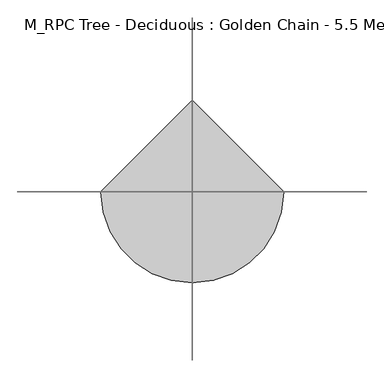
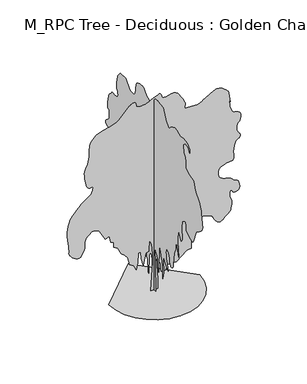
"""IFC4 building model written with IfcOpenShell, lengths in millimetres: geographic element geometry, M_RPC Tree - Deciduous : Golden Chain - 5.5 Meters."""

from ifc_helpers import new_model, si_unit, origin, place, context, project, spatial, triangles, source, transform, mapped, element, save


def m_rpc_tree_deciduous_golden_chain_5_5_meters_6778af60(model_context):
    return source(origin(), model_context, "Body", "Tessellation", [
        triangles([(-0.0021492, 84.2526153, 0.0017055), (-0.0021492, -79.7118042, 0.0017055), (-0.0021492, -55.1171299, 770.634066), (-0.0021492, -30.52271, 1205.1391577), (-0.0021492, -128.9011618, 1090.3648407), (-0.0021492, -161.6941456, 983.7870438), (-0.0021492, -161.6941456, 778.8331295), (-0.0021492, -202.6851937, 614.8669024), (-0.0021492, -227.2798771, 1410.0956154), (-0.0021492, -292.8648273, 1254.3285244), (-0.0021492, -391.2435245, 934.5977497), (-0.0021492, -407.6416878, 557.4810519), (-0.0021492, -448.6319547, 754.2384825), (-0.0021492, -424.0372713, 1123.1586239), (-0.0021492, -399.4426243, 1229.7338047), (-0.0021492, -563.4062716, 1024.7798904), (-0.0021492, -645.3893852, 910.00303), (-0.0021492, -571.6053351, 1164.1488544), (-0.0021492, -566.3701532, 1202.7023878), (-0.0021492, -561.3514189, 1240.6803749), (-0.0021492, -556.7629998, 1277.5125744), (-0.0021492, -552.8187638, 1312.6233673), (-0.0021492, -549.7351948, 1345.442585), (-0.0021492, -547.7261604, 1375.3895943), (-0.0021492, -547.0106518, 1401.8965519), (-0.0021492, -548.2048739, 1425.0576382), (-0.0021492, -551.550709, 1445.6369053), (-0.0021492, -556.6891308, 1464.0644142), (-0.0021492, -563.2636931, 1480.7706619), (-0.0021492, -570.9127539, 1496.1884708), (-0.0021492, -579.2773232, 1510.7457218), (-0.0021492, -588.000955, 1524.870005), (-0.0021492, -615.9185097, 1493.2475166), (-0.0021492, -642.6877333, 1461.6276443), (-0.0021492, -667.1627655, 1430.0051559), (-0.0021492, -688.1976734, 1398.3826675), (-0.0021492, -704.6416552, 1366.7627953), (-0.0021492, -715.3488504, 1335.1403069), (-0.0021492, -719.173399, 1303.5178185), (-0.0021492, -720.8463346, 1273.0922047), (-0.0021492, -725.5315138, 1244.8155876), (-0.0021492, -732.7248247, 1218.3340645), (-0.0021492, -741.9270973, 1193.2836313), (-0.0021492, -752.6342926, 1169.31024), (-0.0021492, -764.3472404, 1146.0549007), (-0.0021492, -776.5592857, 1123.1586239), (-0.0021492, -799.2416948, 1123.4208899), (-0.0021492, -820.9921841, 1125.2618385), (-0.0021492, -840.8787609, 1130.2576818), (-0.0021492, -857.9695055, 1139.9845591), (-0.0021492, -871.3298819, 1156.0210802), (-0.0021492, -880.0305862, 1179.9486168), (-0.0021492, -883.1370827, 1213.3382212), (-0.0021492, -884.8100183, 1255.5711811), (-0.0021492, -889.4951975, 1304.2589069), (-0.0021492, -896.6884357, 1358.3243568), (-0.0021492, -905.890781, 1416.6930325), (-0.0021492, -916.5979763, 1478.2854939), (-0.0021492, -928.3109241, 1542.0320389), (-0.0021492, -940.5255129, 1606.8530823), (-0.0021492, -1006.1104631, 1762.6177025), (-0.0021492, -1030.7051102, 2041.3581013), (-0.0021492, -1137.2829071, 1615.0495296), (-0.0021492, -1096.2900604, 2033.1590378), (-0.0021492, -1120.8847801, 2385.6835957), (-0.0021492, -1260.2563602, 2139.7368347), (-0.0021492, -1270.7241806, 2153.8611179), (-0.0021492, -1280.7616493, 2168.4183689), (-0.0021492, -1289.9410309, 2183.833707), (-0.0021492, -1297.8295029, 2200.5424255), (-0.0021492, -1303.9940975, 2218.9699345), (-0.0021492, -1308.0095501, 2239.5492016), (-0.0021492, -1309.4456543, 2262.7102879), (-0.0021492, -1307.6275967, 2290.0778034), (-0.0021492, -1302.9424175, 2322.033847), (-0.0021492, -1296.538448, 2357.1447853), (-0.0021492, -1289.5590775, 2393.9769848), (-0.0021492, -1283.1526371, 2431.0968121), (-0.0021492, -1278.467458, 2467.0683083), (-0.0021492, -1276.6518711, 2500.45784), (-0.0021492, -1277.8461296, 2532.7959824), (-0.0021492, -1281.1944717, 2566.4375336), (-0.0021492, -1286.3329662, 2601.1435547), (-0.0021492, -1292.9049488, 2636.6899315), (-0.0021492, -1300.5540459, 2672.8981865), (-0.0021492, -1308.9185062, 2709.5395546), (-0.0021492, -1317.642247, 2746.4096878), (-0.0021492, -1349.0965771, 2763.5973015), (-0.0021492, -1379.5477707, 2778.4931946), (-0.0021492, -1407.98993, 2788.7800667), (-0.0021492, -1433.4222439, 2792.1923584), (-0.0021492, -1454.8366344, 2786.4374771), (-0.0021492, -1471.2347614, 2769.1992851), (-0.0021492, -1481.6057854, 2738.2107697), (-0.0021492, -1484.4041611, 2701.900486), (-0.0021492, -1481.8935585, 2669.6135033), (-0.0021492, -1478.8100258, 2640.3309883), (-0.0021492, -1479.8871403, 2613.0602692), (-0.0021492, -1489.8532471, 2586.7825127), (-0.0021492, -1513.444685, 2560.5300453), (-0.0021492, -1555.3924152, 2533.2517685), (-0.0021492, -1606.8988644, 2505.0718025), (-0.0021492, -1655.253035, 2478.4681938), (-0.0021492, -1699.3015091, 2456.025087), (-0.0021492, -1737.903368, 2440.3219757), (-0.0021492, -1769.9076645, 2433.9411152), (-0.0021492, -1794.1662128, 2439.4615631), (-0.0021492, -1809.5357689, 2459.4676094), (-0.0021492, -1957.1037964, 2820.1761154), (-0.0021492, -2096.4727604, 2918.5648773), (-0.0021492, -2133.9033245, 2947.2108032), (-0.0021492, -2168.0337994, 2976.9770096), (-0.0021492, -2197.5760368, 3008.067263), (-0.0021492, -2221.2386913, 3040.5580124), (-0.0021492, -2237.731144, 3074.6530243), (-0.0021492, -2245.7620491, 3110.453746), (-0.0021492, -2244.0407879, 3148.1136566), (-0.0021492, -2235.2459759, 3194.9398682), (-0.0021492, -2223.869054, 3254.6760475), (-0.0021492, -2211.3438011, 3322.1530334), (-0.0021492, -2199.1063213, 3392.2013741), (-0.0021492, -2188.5901028, 3459.67836), (-0.0021492, -2181.2287788, 3519.4145393), (-0.0021492, -2178.4558376, 3566.2154617), (-0.0021492, -2170.3281361, 3608.6875786), (-0.0021492, -2147.5744377, 3658.060437), (-0.0021492, -2112.6315125, 3713.1367264), (-0.0021492, -2067.9338047, 3772.8217461), (-0.0021492, -2015.9257874, 3835.9446373), (-0.0021492, -1959.038998, 3901.3845383), (-0.0021492, -1899.7152935, 3967.9447197), (-0.0021492, -1842.3294067, 4197.4932083), (-0.0021492, -1629.1739582, 4246.6875893), (-0.0021492, -1457.0136818, 4328.652935), (-0.0021492, -1458.3505188, 4335.1970123), (-0.0021492, -1461.6963902, 4352.7409996), (-0.0021492, -1466.0480141, 4378.3565872), (-0.0021492, -1470.3970219, 4408.9631493), (-0.0021492, -1473.7428932, 4441.6065056), (-0.0021492, -1475.082201, 4473.2060303), (-0.0021492, -1473.409338, 4500.8334137), (-0.0021492, -1467.7438408, 4526.8565346), (-0.0021492, -1458.2079403, 4555.4515915), (-0.0021492, -1445.4433125, 4586.2107605), (-0.0021492, -1430.0993362, 4618.7015099), (-0.0021492, -1412.8176876, 4652.4654373), (-0.0021492, -1394.2474548, 4687.1205894), (-0.0021492, -1375.0306046, 4722.1829842), (-0.0021492, -1342.2368214, 4918.9352188), (-0.0021492, -1448.8146183, 5009.1250626), (-0.0021492, -1579.9871349, 4984.5277267), (-0.0021492, -1653.7685326, 4877.9400467), (-0.0021492, -1653.7685326, 4976.3288086), (-0.0021492, -1538.9942883, 5082.8914902), (-0.0021492, -1350.4358849, 5107.488826), (-0.0021492, -1202.8678574, 5074.692572), (-0.0021492, -1055.2998299, 5156.6829163), (-0.0021492, -948.7220329, 5164.8818344), (-0.0021492, -940.8819592, 5161.1390396), (-0.0021492, -920.1372952, 5151.1065125), (-0.0021492, -890.6409851, 5136.4911255), (-0.0021492, -856.5588358, 5118.9980072), (-0.0021492, -822.0437914, 5100.3334488), (-0.0021492, -791.2590425, 5082.280481), (-0.0021492, -768.3627657, 5066.4930725), (-0.0021492, -752.5400396, 5050.8591431), (-0.0021492, -739.1541561, 5033.7985565), (-0.0021492, -726.6289759, 5017.8844116), (-0.0021492, -713.3882143, 5005.6874817), (-0.0021492, -697.8532614, 4999.805864), (-0.0021492, -678.4453617, 5002.8359116), (-0.0021492, -653.5859053, 5017.2989822), (-0.0021492, -627.1527803, 5039.5790176), (-0.0021492, -603.7294281, 5064.0234558), (-0.0021492, -582.814135, 5090.2247635), (-0.0021492, -563.9078762, 5117.8777267), (-0.0021492, -546.5090472, 5146.6253906), (-0.0021492, -530.1108839, 5176.0602219), (-0.0021492, -514.2169049, 5205.8775879), (-0.0021492, -415.8382078, 5410.8290314), (-0.0021492, -169.8924643, 5451.8242035), (-0.0021492, -163.845268, 5451.6713058), (-0.0021492, -147.6161895, 5450.6783432), (-0.0021492, -124.0728773, 5447.9540909), (-0.0021492, -96.0842423, 5442.6323227), (-0.0021492, -66.5181736, 5433.8985535), (-0.0021492, -38.2425694, 5420.8359787), (-0.0021492, -14.1260625, 5402.6295319), (-0.0021492, 3.3458589, 5384.2457703), (-0.0021492, 15.2248406, 5370.0373352), (-0.0021492, 23.9488607, 5358.0950409), (-0.0021492, 31.9557643, 5346.6114395), (-0.0021492, 41.6836339, 5333.6761826), (-0.0021492, 55.5706269, 5317.4306625), (-0.0021492, 76.0543103, 5296.0418518), (-0.0021492, 97.13535, 5271.2916183), (-0.0021492, 113.1971331, 5247.5349289), (-0.0021492, 127.2514169, 5226.7827072), (-0.0021492, 142.3091915, 5211.0464584), (-0.0021492, 161.3827366, 5202.3638489), (-0.0021492, 187.483033, 5202.6946426), (-0.0021492, 223.6221062, 5214.076506), (-0.0021492, 264.351397, 5233.7851868), (-0.0021492, 302.4974698, 5257.3889786), (-0.0021492, 338.4919115, 5284.2012955), (-0.0021492, 372.7676173, 5313.5855484), (-0.0021492, 405.7523409, 5344.9307281), (-0.0021492, 437.8763975, 5377.549086), (-0.0021492, 469.5675954, 5410.8290314), (-0.0021492, 492.466452, 5419.4860611), (-0.0021492, 515.7217913, 5427.3286057), (-0.0021492, 539.6951463, 5433.618338), (-0.0021492, 564.7456158, 5437.5396103), (-0.0021492, 591.2271026, 5438.3035172), (-0.0021492, 619.503756, 5435.1205719), (-0.0021492, 649.9294424, 5427.2268677), (-0.0021492, 681.4067362, 5417.9076691), (-0.0021492, 712.0259428, 5409.8610672), (-0.0021492, 740.9213448, 5401.4075134), (-0.0021492, 767.2373257, 5390.7895569), (-0.0021492, 790.1107115, 5376.3009064), (-0.0021492, 808.6833424, 5356.2364334), (-0.0021492, 822.0921896, 5328.8381058), (-0.0021492, 831.6764156, 5297.4679276), (-0.0021492, 839.5393805, 5266.5047012), (-0.0021492, 845.9687845, 5235.9240097), (-0.0021492, 851.2523283, 5205.5973724), (-0.0021492, 855.672698, 5175.5253708), (-0.0021492, 859.522681, 5145.5556885), (-0.0021492, 863.0824202, 5115.6877441), (-0.0021492, 868.5086151, 5085.9976959), (-0.0021492, 874.8667299, 5057.4029297), (-0.0021492, 883.0886845, 5030.9469864), (-0.0021492, 894.1065439, 5007.6989868), (-0.0021492, 908.8546263, 4988.7803741), (-0.0021492, 928.2625259, 4975.2085281), (-0.0021492, 953.2646336, 4968.1298904), (-0.0021492, 983.5706326, 4964.7940475), (-0.0021492, 1017.0340696, 4962.6296448), (-0.0021492, 1051.7859455, 4962.7313828), (-0.0021492, 1085.9648186, 4966.2962814), (-0.0021492, 1117.7069944, 4974.4446213), (-0.0021492, 1145.1458719, 4988.347261), (-0.0021492, 1166.4176113, 5009.1250626), (-0.0021492, 1187.9516893, 5037.6180908), (-0.0021492, 1215.2250246, 5071.5857849), (-0.0021492, 1244.9327316, 5107.4120865), (-0.0021492, 1273.7822788, 5141.5326782), (-0.0021492, 1298.4736496, 5170.3309204), (-0.0021492, 1315.7070454, 5190.2430771), (-0.0021492, 1322.1822315, 5197.6786697), (-0.0021492, 1576.328056, 5181.2802521), (-0.0021492, 1674.7067894, 5058.2941544), (-0.0021492, 1679.9878624, 5049.3057495), (-0.0021492, 1685.3426228, 5039.1203247), (-0.0021492, 1690.840107, 5026.4652832), (-0.0021492, 1696.5540024, 5010.1691849), (-0.0021492, 1702.550584, 4988.9838501), (-0.0021492, 1708.9086262, 4961.7134216), (-0.0021492, 1715.69702, 4927.1347183), (-0.0021492, 1722.2461842, 4888.9655365), (-0.0021492, 1727.9344997, 4851.6622902), (-0.0021492, 1732.907452, 4815.0465019), (-0.0021492, 1737.304858, 4779.0417229), (-0.0021492, 1741.2720577, 4743.4444771), (-0.0021492, 1744.9539551, 4708.1530266), (-0.0021492, 1748.4908031, 4672.9886032), (-0.0021492, 1731.0893944, 4648.3403984), (-0.0021492, 1714.6937382, 4623.4122688), (-0.0021492, 1700.3046455, 4597.9237083), (-0.0021492, 1688.927869, 4571.5442139), (-0.0021492, 1681.5665451, 4544.0441483), (-0.0021492, 1679.2239555, 4515.0927177), (-0.0021492, 1682.9058529, 4484.4352867), (-0.0021492, 1691.9172215, 4457.546521), (-0.0021492, 1704.798848, 4438.9584114), (-0.0021492, 1721.4109154, 4426.9908279), (-0.0021492, 1741.6082291, 4419.8866104), (-0.0021492, 1765.2454491, 4415.940049), (-0.0021492, 1792.1827583, 4413.4445618), (-0.0021492, 1822.2748169, 4410.6435699), (-0.0021492, 1851.5776794, 4410.5162521), (-0.0021492, 1877.0099934, 4414.7177399), (-0.0021492, 1899.7152935, 4419.453788), (-0.0021492, 1920.8445271, 4421.0580505), (-0.0021492, 1941.543409, 4415.7871513), (-0.0021492, 1962.9576542, 4399.8982956), (-0.0021492, 1986.2385006, 4369.6483978), (-0.0021492, 2009.8529022, 4339.016256), (-0.0021492, 2031.6033188, 4320.2755394), (-0.0021492, 2051.6324741, 4307.2641243), (-0.0021492, 2070.0854176, 4293.8451759), (-0.0021492, 2087.1024021, 4273.8057014), (-0.0021492, 2102.8308025, 4241.0094475), (-0.0021492, 2117.4110172, 4189.2939995), (-0.0021492, 2130.4606567, 4132.1297562), (-0.0021492, 2141.5040234, 4085.4561516), (-0.0021492, 2150.5382103, 4046.6759605), (-0.0021492, 2157.565979, 4013.1922485), (-0.0021492, 2162.5848587, 3982.4330795), (-0.0021492, 2165.5945587, 3951.8009377), (-0.0021492, 2166.6003113, 3918.7500481), (-0.0021492, 2163.9699486, 3888.1437767), (-0.0021492, 2156.6086246, 3865.7361328), (-0.0021492, 2145.3030647, 3850.1274925), (-0.0021492, 2130.8426102, 3839.9676476), (-0.0021492, 2114.0167477, 3833.9075523), (-0.0021492, 2095.6120571, 3830.5464203), (-0.0021492, 2076.4181705, 3828.5602043), (-0.0021492, 2076.4181705, 3615.4098427), (-0.0021492, 2076.5861835, 3611.7687859), (-0.0021492, 2077.7574783, 3607.2362137), (-0.0021492, 2080.9351913, 3600.9979317), (-0.0021492, 2087.1278366, 3592.1877136), (-0.0021492, 2097.3334637, 3579.9143349), (-0.0021492, 2112.5576797, 3563.3636009), (-0.0021492, 2133.8065281, 3541.6437057), (-0.0021492, 2158.6890209, 3518.8288193), (-0.0021492, 2183.2835953, 3498.7640556), (-0.0021492, 2206.2996323, 3480.0997879), (-0.0021492, 2226.4484024, 3461.6134163), (-0.0021492, 2242.4391415, 3441.9561859), (-0.0021492, 2252.9807945, 3419.8796265), (-0.0021492, 2256.7799812, 3394.0602722), (-0.0021492, 2250.3276134, 3369.7687317), (-0.0021492, 2232.2566235, 3352.3773514), (-0.0021492, 2204.5070091, 3340.7152725), (-0.0021492, 2169.0142628, 3333.6366348), (-0.0021492, 2127.7106792, 3329.995578), (-0.0021492, 2082.5368378, 3328.6715309), (-0.0021492, 2035.4277946, 3328.4677643), (-0.0021492, 2021.5658501, 3329.995578), (-0.0021492, 2008.8496204, 3330.1737648), (-0.0021492, 1998.4275822, 3327.6274086), (-0.0021492, 1991.4508278, 3320.9815933), (-0.0021492, 1989.05984, 3308.886692), (-0.0021492, 1992.405566, 3289.9677887), (-0.0021492, 2002.6366276, 3262.9005455), (-0.0021492, 2020.3945553, 3234.9676575), (-0.0021492, 2044.3195484, 3213.2224731), (-0.0021492, 2072.5477673, 3195.7802238), (-0.0021492, 2103.212756, 3180.7570129), (-0.0021492, 2134.4508202, 3166.3195221), (-0.0021492, 2164.4003002, 3150.6088531), (-0.0021492, 2191.195031, 3131.7155296), (-0.0021492, 2214.6667088, 3115.4700096), (-0.0021492, 2235.4113728, 3106.0996513), (-0.0021492, 2252.7159851, 3099.4538361), (-0.0021492, 2265.8625664, 3091.381945), (-0.0021492, 2274.1329918, 3077.7083611), (-0.0021492, 2276.8091366, 3054.2824654), (-0.0021492, 2273.1754921, 3016.9539299), (-0.0021492, 2263.7593517, 2975.5765137), (-0.0021492, 2250.0398403, 2941.939904), (-0.0021492, 2232.735228, 2914.7709229), (-0.0021492, 2212.5634941, 2892.7455231), (-0.0021492, 2190.2375313, 2874.6158157), (-0.0021492, 2166.4806965, 2859.0580444), (-0.0021492, 2142.0055916, 2844.7731606), (-0.0021492, 2133.3761765, 2827.1783043), (-0.0021492, 2125.6812973, 2809.2779434), (-0.0021492, 2119.8477871, 2790.7918625), (-0.0021492, 2116.8125072, 2771.4654259), (-0.0021492, 2117.5051975, 2750.9675491), (-0.0021492, 2122.8599579, 2729.044178), (-0.0021492, 2133.8065281, 2705.4145157), (-0.0021492, 2153.6931049, 2682.9815826), (-0.0021492, 2182.4714355, 2663.4005104), (-0.0021492, 2215.980582, 2644.532476), (-0.0021492, 2250.062804, 2624.2386566), (-0.0021492, 2280.5623959, 2600.3543587), (-0.0021492, 2303.3160942, 2570.7407593), (-0.0021492, 2314.1683388, 2533.2517685), (-0.0021492, 2316.6306885, 2491.7827881), (-0.0021492, 2316.7960854, 2450.4562408), (-0.0021492, 2314.3822792, 2407.4085777), (-0.0021492, 2309.1012062, 2360.7782845), (-0.0021492, 2300.6627678, 2308.6964344), (-0.0021492, 2288.7842777, 2249.3015133), (-0.0021492, 2273.1754921, 2180.7272106), (-0.0021492, 2256.9479942, 2122.3126076), (-0.0021492, 2242.7269146, 2087.8459614), (-0.0021492, 2229.5091167, 2067.1470795), (-0.0021492, 2216.2913189, 2050.0334438), (-0.0021492, 2202.0702393, 2026.3248619), (-0.0021492, 2185.8401253, 1985.8335835), (-0.0021492, 2166.6003113, 1918.3847935), (-0.0021492, 2149.5808559, 1842.5203835), (-0.0021492, 2138.8736607, 1783.2936207), (-0.0021492, 2131.7517117, 1740.2713921), (-0.0021492, 2125.4903206, 1713.0234913), (-0.0021492, 2117.362619, 1701.1195667), (-0.0021492, 2104.6463894, 1704.1317375), (-0.0021492, 2084.617234, 1721.6273266), (-0.0021492, 2060.5012642, 1758.0775726), (-0.0021492, 2037.2458523, 1813.4570412), (-0.0021492, 2014.7060944, 1880.5977104), (-0.0021492, 1992.7391212, 1952.324437), (-0.0021492, 1971.2051159, 2021.4716698), (-0.0021492, 1949.9562675, 2080.8664455), (-0.0021492, 1928.8526138, 2123.3387077), (-0.0021492, 1903.2291779, 2154.4824463), (-0.0021492, 1869.4322582, 2184.7680977), (-0.0021492, 1828.8238358, 2214.3331535), (-0.0021492, 1782.7664726, 2243.3252792), (-0.0021492, 1732.6196789, 2271.8870533), (-0.0021492, 1679.7509583, 2300.1636703), (-0.0021492, 1625.51735, 2328.2952381), (-0.0021492, 1580.1042789, 2357.6693172), (-0.0021492, 1536.2697453, 2384.1049129), (-0.0021492, 1495.5901062, 2404.6612164), (-0.0021492, 1459.6414284, 2416.3971279), (-0.0021492, 1430.0025398, 2416.3715481), (-0.0021492, 1408.2521233, 2401.6489002), (-0.0021492, 1395.9662453, 2369.2854687), (-0.0021492, 1387.7442181, 2327.3633183), (-0.0021492, 1377.3731941, 2285.8713741), (-0.0021492, 1365.2069309, 2244.7359489), (-0.0021492, 1351.6071796, 2203.8882969), (-0.0021492, 1336.9303139, 2163.2544399), (-0.0021492, 1321.5379395, 2122.7657776), (-0.0021492, 1305.7865753, 2082.3484772), (-0.0021492, 1125.4248373, 1926.583857), (-0.0021492, 1107.9775738, 1907.1276318), (-0.0021492, 1091.2458916, 1886.8820652), (-0.0021492, 1075.9502409, 1865.0602867), (-0.0021492, 1062.8037323, 1840.8729549), (-0.0021492, 1052.5268887, 1813.5282578), (-0.0021492, 1045.8352186, 1782.2419407), (-0.0021492, 1043.4442308, 1746.2220463), (-0.0021492, 1042.7261787, 1711.1595062), (-0.0021492, 1040.7196878, 1682.5468632), (-0.0021492, 1037.6361551, 1659.3168858), (-0.0021492, 1033.6919191, 1640.3851925), (-0.0021492, 1029.1035364, 1624.6822266), (-0.0021492, 1024.0847294, 1611.1308735), (-0.0021492, 1018.8495838, 1598.6540188), (-0.0021492, 871.2814837, 1500.2752853), (-0.0021492, 854.8859001, 1328.1125381), (-0.0021492, 731.9125196, 1270.7241806), (-0.0021492, 699.1188091, 1057.5711302), (-0.0021492, 567.9463288, 1024.7798904), (-0.0021492, 579.9928319, 1019.3537682), (-0.0021492, 590.5345213, 1012.9956533), (-0.0021492, 598.0638946, 1004.7736261), (-0.0021492, 601.0736309, 993.7558393), (-0.0021492, 598.0638946, 979.0076843), (-0.0021492, 587.5222415, 959.5997847), (-0.0021492, 567.9463288, 934.5977497), (-0.0021492, 544.3090362, 908.8801334), (-0.0021492, 522.3905339, 887.4631994), (-0.0021492, 501.9081359, 869.6340551), (-0.0021492, 482.5715618, 854.6720324), (-0.0021492, 464.0956183, 841.8616224), (-0.0021492, 446.192605, 830.4822298), (-0.0021492, 428.5773285, 819.8234327), (-0.0021492, 416.3169213, 852.4974558), (-0.0021492, 404.2703819, 880.9396151), (-0.0021492, 392.6541942, 900.9203722), (-0.0021492, 381.6821895, 908.2104795), (-0.0021492, 371.5733952, 898.5777826), (-0.0021492, 362.5365921, 867.7931065), (-0.0021492, 354.7933147, 811.6243692), (-0.0021492, 347.289376, 757.5588467), (-0.0021492, 338.9222268, 728.4470335), (-0.0021492, 329.8396053, 713.1030573), (-0.0021492, 320.1840537, 700.3409729), (-0.0021492, 310.0981504, 678.9725098), (-0.0021492, 299.7245467, 637.8141209), (-0.0021492, 289.2083463, 565.677572), (-0.0021492, 280.1002358, 485.3215393), (-0.0021492, 273.5766333, 424.7553234), (-0.0021492, 269.2021002, 380.6814875), (-0.0021492, 266.5488464, 349.8000149), (-0.0021492, 265.1865749, 328.815976), (-0.0021492, 264.6849704, 314.426847), (-0.0021492, 264.613663, 303.3351912), (-0.0021492, 240.0187434, 811.6243692), (-0.0021492, 227.6618124, 844.6574547), (-0.0021492, 214.9461096, 875.6102165), (-0.0021492, 201.5133903, 902.4023312), (-0.0021492, 187.005355, 922.9585619), (-0.0021492, 171.062996, 935.1961143), (-0.0021492, 153.328032, 937.037063), (-0.0021492, 133.4419729, 926.401157), (-0.0021492, 115.707018, 904.291678), (-0.0021492, 103.9950694, 874.0085701), (-0.0021492, 97.3026454, 836.9141773), (-0.0021492, 94.6257194, 794.3680824), (-0.0021492, 94.9603011, 747.7377892), (-0.0021492, 97.3026454, 698.3803368), (-0.0021492, 100.6487348, 647.6606855), (-0.0021492, 84.2526153, 237.7499866), (88.4435659, 0.0002505, 0.0), (-86.3932913, 0.0002505, 0.0), (-44.7656723, 0.0002025, 807.5807934), (-36.4400473, 0.0001919, 1032.3704155), (-69.7422955, 0.0001759, 1307.1158546), (-128.0216733, 0.0001652, 1448.6490761), (-144.6726646, 0.0001865, 1140.6032713), (-227.9278935, 0.0001865, 1115.6266708), (-294.532658, 0.0002025, 799.2544121), (-352.8122947, 0.0001919, 999.0699772), (-361.138676, 0.0001812, 1182.2301636), (-427.7421324, 0.0001812, 1182.2301636), (-444.3923879, 0.0001972, 915.8137218), (-486.0217873, 0.0002079, 732.6509193), (-552.6252437, 0.0002025, 874.1842861), (-660.8581358, 0.0001972, 940.7903223), (-702.4849554, 0.0001812, 1157.2534904), (-785.7412107, 0.0001759, 1257.1625084), (-877.3238474, 0.0001759, 1332.0923824), (-977.2303219, 0.0001599, 1523.5789501), (-1085.4632504, 0.0001599, 1581.8586777), (-1085.4632504, 0.0001492, 1723.3945152), (-1160.3931244, 0.0001492, 1748.3711884), (-1202.019944, 0.0001386, 1939.857756), (-1318.5792538, 0.0001386, 1889.9044098), (-1468.4390018, 0.0001226, 2172.9736141), (-1502.3250149, 0.0001226, 2194.0442757), (-1536.1347244, 0.0001226, 2213.0727654), (-1569.8018555, 0.0001173, 2228.0246143), (-1603.2501045, 0.0001173, 2236.8602669), (-1636.4053482, 0.0001173, 2237.5401672), (-1669.1991314, 0.0001173, 2228.0246143), (-1701.5548599, 0.0001226, 2206.2766685), (-1733.4726791, 0.0001226, 2179.018594), (-1764.2269066, 0.0001226, 2153.3621658), (-1792.651189, 0.0001279, 2127.850787), (-1817.579464, 0.0001279, 2101.0306217), (-1837.8479942, 0.0001279, 2071.4426022), (-1852.2879559, 0.0001332, 2037.6304218), (-1859.7409893, 0.0001332, 1998.1373383), (-1862.0709343, 0.0001386, 1954.9318359), (-1863.0894768, 0.0001386, 1911.4359444), (-1864.5459286, 0.0001439, 1868.3754913), (-1868.1871307, 0.0001439, 1826.4812462), (-1875.759779, 0.0001439, 1786.4790367), (-1889.0133305, 0.0001492, 1749.0993416), (-1909.6943356, 0.0001492, 1715.0681339), (-1930.6655846, 0.0001546, 1683.7079842), (-1945.9586918, 0.0001546, 1654.8226833), (-1959.0644325, 0.0001546, 1629.87159), (-1973.4840466, 0.0001546, 1610.3057785), (-1992.7085999, 0.0001599, 1597.5870781), (-2020.2341, 0.0001599, 1593.1693245), (-2059.5539383, 0.0001599, 1598.5088242), (-2106.0849644, 0.0001546, 1614.4818317), (-2151.4523987, 0.0001546, 1639.6289886), (-2193.4662586, 0.0001546, 1671.9108845), (-2229.9496422, 0.0001492, 1709.2905796), (-2258.7125668, 0.0001492, 1749.7308437), (-2277.5730434, 0.0001439, 1791.1870342), (-2284.3435604, 0.0001439, 1831.6274437), (-2284.0049183, 0.0001439, 1867.2347179), (-2283.6662762, 0.0001386, 1899.34613), (-2284.3435604, 0.0001386, 1933.6447632), (-2287.0630165, 0.0001332, 1975.8062885), (-2292.8405708, 0.0001332, 2031.5116093), (-2302.6947659, 0.0001279, 2106.4440994), (-2317.6466148, 0.0001226, 2206.2766685), (-2328.3767738, 0.0001119, 2318.4664776), (-2327.0169731, 0.0001066, 2424.8304794), (-2316.773267, 0.0001013, 2522.6006744), (-2300.8512737, 9.59e-05, 2609.0116791), (-2282.4516701, 9.06e-05, 2681.301162), (-2264.780365, 9.06e-05, 2736.6829559), (-2251.0431221, 8.53e-05, 2772.4075195), (-2228.7604706, 8.53e-05, 2807.0370918), (-2187.9815643, 7.99e-05, 2856.639006), (-2135.6984184, 7.99e-05, 2914.8473717), (-2078.9007225, 7.46e-05, 2975.2454292), (-2024.5780209, 7.46e-05, 3031.4167099), (-1979.7200031, 6.93e-05, 3076.9444542), (-1951.3211552, 6.93e-05, 3105.4374825), (-1924.2819626, 6.4e-05, 3127.0812195), (-1882.823156, 6.4e-05, 3155.2940323), (-1832.9183533, 6.4e-05, 3188.4469505), (-1780.5385563, 5.86e-05, 3224.9607101), (-1731.6521507, 5.86e-05, 3263.2060501), (-1692.2328999, 5.33e-05, 3301.6042877), (-1668.2519508, 5.33e-05, 3338.5511604), (-1656.1646072, 5.33e-05, 3371.3218346), (-1648.0088551, 4.8e-05, 3398.84748), (-1643.1300831, 4.8e-05, 3421.9931602), (-1640.8716454, 4.8e-05, 3441.6759705), (-1640.5812561, 4.8e-05, 3458.7106865), (-1641.5997986, 4.8e-05, 3473.988533), (-1643.2752777, 4.26e-05, 3488.4260239), (-1673.4947994, 4.26e-05, 3483.4862091), (-1703.0597099, 4.26e-05, 3481.1180397), (-1731.3135086, 4.26e-05, 3483.8172935), (-1757.6014389, 4.26e-05, 3494.1806145), (-1781.2667095, 4.26e-05, 3514.7546494), (-1801.6574707, 4.26e-05, 3548.0601746), (-1818.1141697, 3.73e-05, 3596.6435463), (-1832.6281094, 3.2e-05, 3658.2386238), (-1846.5614159, 3.2e-05, 3726.3519081), (-1858.3075012, 2.66e-05, 3797.4190819), (-1866.2698059, 2.13e-05, 3867.7223488), (-1868.8440674, 1.6e-05, 3933.671521), (-1864.4261684, 1.6e-05, 3991.625251), (-1851.414608, 1.07e-05, 4037.8913223), (-1831.8514126, 1.07e-05, 4080.6180748), (-1810.1034668, 5.3e-06, 4129.8889046), (-1788.0628063, 5.3e-06, 4185.1436714), (-1767.626263, 0.0, 4245.7710754), (-1750.6831112, -5.3e-06, 4311.2106857), (-1739.1280025, -1.07e-05, 4380.8773636), (-1734.8579144, -1.07e-05, 4454.1853889), (-1735.4894165, -1.6e-05, 4523.877356), (-1735.8280586, -2.13e-05, 4584.5303398), (-1733.5466572, -2.13e-05, 4638.3334511), (-1726.3125057, -2.66e-05, 4687.5025429), (-1711.7987114, -3.2e-05, 4734.1761475), (-1687.6699516, -3.2e-05, 4780.5442474), (-1651.601659, -3.73e-05, 4828.8218239), (-1604.6581581, -3.73e-05, 4875.2407928), (-1551.3056007, -4.26e-05, 4914.6575729), (-1494.3144573, -4.26e-05, 4947.2247711), (-1436.4472046, -4.26e-05, 4973.1202835), (-1380.4746037, -4.26e-05, 4992.421431), (-1329.161602, -4.8e-05, 5005.3566879), (-1285.2761993, -4.8e-05, 5012.0022125), (-1238.819006, -4.8e-05, 5019.8197586), (-1181.7285227, -4.8e-05, 5034.7665207), (-1119.6854347, -4.8e-05, 5054.8059952), (-1058.3731888, -4.8e-05, 5077.9260956), (-1003.4673832, -5.33e-05, 5102.03974), (-960.651392, -5.33e-05, 5125.1598404), (-935.6009588, -5.33e-05, 5145.1993149), (-669.1845171, -6.93e-05, 5428.27099), (-646.0030106, -6.93e-05, 5444.1601364), (-622.8954094, -7.46e-05, 5458.928421), (-599.9328938, -7.46e-05, 5471.5328842), (-577.1893693, -7.46e-05, 5480.8520828), (-554.7386684, -7.46e-05, 5485.7918976), (-532.6495734, -7.46e-05, 5485.2826263), (-510.9983877, -7.46e-05, 5478.2295685), (-495.8275477, -7.46e-05, 5462.4933197), (-489.5407585, -6.93e-05, 5439.0418442), (-486.7500132, -6.93e-05, 5411.3888809), (-482.064834, -6.93e-05, 5382.9725922), (-470.0972506, -6.93e-05, 5357.3567139), (-445.4618357, -6.4e-05, 5337.9794083), (-402.7655319, -6.4e-05, 5328.3544144), (-352.1553217, -6.4e-05, 5326.9794983), (-306.7905035, -6.4e-05, 5329.5258545), (-265.7951497, -6.4e-05, 5335.3568939), (-228.2925333, -6.4e-05, 5343.8104477), (-193.4123404, -6.4e-05, 5354.2249283), (-160.2801876, -6.93e-05, 5365.9375854), (-128.0216733, -6.93e-05, 5378.3124115), (-76.4902348, -6.93e-05, 5408.3588333), (-26.1968067, -6.93e-05, 5436.7501236), (21.6206779, -7.46e-05, 5461.7805725), (65.7244948, -7.46e-05, 5481.7688873), (104.8766017, -7.46e-05, 5495.0605179), (137.8389157, -7.46e-05, 5500.0003326), (163.3739486, -7.46e-05, 5494.8820404), (179.7578323, -7.46e-05, 5482.2525787), (188.4231282, -7.46e-05, 5466.2872742), (192.8648993, -7.46e-05, 5447.6994553), (196.5786624, -6.93e-05, 5427.2012878), (203.0594986, -6.93e-05, 5405.5578415), (215.8026888, -6.93e-05, 5383.4562836), (238.3035501, -6.93e-05, 5361.6599396), (275.7078804, -6.4e-05, 5352.0093658), (327.5301169, -6.93e-05, 5359.8263306), (388.8194718, -6.93e-05, 5376.0974304), (454.6234131, -6.93e-05, 5391.7569397), (519.9893723, -6.93e-05, 5397.8426147), (579.9673974, -6.93e-05, 5385.2643127), (629.6048836, -6.4e-05, 5345.0068863), (669.510442, -6.4e-05, 5289.625383), (704.1731518, -5.86e-05, 5237.2989258), (734.4638901, -5.86e-05, 5187.5188248), (761.2611643, -5.33e-05, 5139.7758087), (785.4382496, -5.33e-05, 5093.5606064), (807.8660231, -4.8e-05, 5048.3633652), (829.420376, -4.8e-05, 5003.6759766), (821.0939947, -3.73e-05, 4853.8011131), (1104.163199, -3.73e-05, 4837.1483505), (1130.912075, -3.73e-05, 4839.0834068), (1157.5870457, -3.73e-05, 4841.7826607), (1184.116967, -3.73e-05, 4846.1111755), (1210.4303318, -3.73e-05, 4852.8334396), (1236.4509819, -3.73e-05, 4862.7639381), (1262.10741, -3.73e-05, 4876.6921577), (1287.3259289, -3.73e-05, 4895.433165), (1317.642247, -4.26e-05, 4918.5532654), (1357.5732399, -4.26e-05, 4944.7039948), (1405.5097034, -4.26e-05, 4973.4260788), (1459.8579849, -4.8e-05, 5004.1852478), (1519.010915, -4.8e-05, 5036.4722305), (1581.3671379, -4.8e-05, 5069.7527573), (1645.3250072, -5.33e-05, 5103.5675537), (1684.4540142, -5.33e-05, 5099.8497574), (1722.8521065, -5.33e-05, 5095.2663162), (1759.7963631, -5.33e-05, 5088.9515854), (1794.5558693, -4.8e-05, 5079.9887604), (1826.3998558, -4.8e-05, 5067.5371948), (1854.6051109, -4.8e-05, 5050.7062454), (1878.4410107, -4.8e-05, 5028.6552658), (1900.2143909, -4.8e-05, 5007.1897156), (1922.1329659, -4.26e-05, 4990.5372437), (1943.3232422, -4.26e-05, 4975.3358459), (1962.9118721, -4.26e-05, 4958.2502609), (1980.023037, -4.26e-05, 4935.9190659), (1993.7857143, -3.73e-05, 4905.0069992), (2003.3267017, -3.73e-05, 4862.1273491), (2036.62714, -2.13e-05, 4620.6877258), (2031.3358932, -2.66e-05, 4643.2223969), (2026.4088684, -2.66e-05, 4661.7340576), (2022.2099968, -2.66e-05, 4672.2502762), (2019.1035004, -2.66e-05, 4670.7477516), (2017.450985, -2.66e-05, 4653.2293442), (2017.6216141, -2.13e-05, 4615.6714622), (2019.9769936, -2.13e-05, 4554.0766754), (2029.0544918, -1.6e-05, 4483.8242775), (2046.7257969, -1.07e-05, 4423.1715843), (2069.3470905, -5.3e-06, 4372.5511276), (2093.2796413, -5.3e-06, 4332.4213097), (2114.8825378, -5.3e-06, 4303.2408234), (2130.5141418, -5.3e-06, 4285.3913315), (2136.5336872, 0.0, 4279.3565254), (2147.5539448, 0.0, 4280.1460121), (2175.7593452, 0.0, 4279.6367409), (2213.8671936, 0.0, 4273.4493279), (2254.5977016, 0.0, 4257.2038078), (2290.6659943, 0.0, 4226.5463768), (2314.794754, 5.3e-06, 4177.0973602), (2319.6963444, 1.07e-05, 4104.5023727), (2308.0216209, 1.07e-05, 4035.0650414), (2289.5024025, 1.6e-05, 3991.3959045), (2267.4871765, 1.6e-05, 3963.6159142), (2245.3241398, 1.6e-05, 3941.7939903), (2226.3694828, 2.13e-05, 3916.0255051), (2213.96399, 2.13e-05, 3876.4308289), (2211.466032, 2.66e-05, 3813.104171), (2219.5963497, 2.66e-05, 3747.2826073), (2234.7188278, 3.2e-05, 3702.4167412), (2253.6250866, 3.2e-05, 3671.9886566), (2273.1169201, 3.73e-05, 3649.4284058), (2289.9862392, 3.73e-05, 3628.141333), (2301.0320766, 3.73e-05, 3601.6598099), (2303.0461979, 4.26e-05, 3563.3380211), (2294.2843781, 4.26e-05, 3529.0395332), (2276.7837021, 4.26e-05, 3512.233873), (2253.0190189, 4.26e-05, 3502.8382256), (2225.4707005, 4.26e-05, 3490.8194824), (2196.6083633, 4.8e-05, 3466.1204086), (2168.9148502, 4.8e-05, 3418.7340569), (2144.8600685, 5.33e-05, 3338.5511604), (2129.882785, 5.86e-05, 3243.8796135), (2124.958231, 6.4e-05, 3160.284716), (2125.8545425, 6.93e-05, 3088.6321129), (2128.3549713, 7.46e-05, 3029.812738), (2128.2327404, 7.46e-05, 2984.6666565), (2121.2660145, 7.46e-05, 2954.0856743), (2103.2331036, 7.99e-05, 2938.9351456), (2080.3674934, 7.99e-05, 2933.5625084), (2059.979203, 7.99e-05, 2930.6853584), (2039.4433926, 7.99e-05, 2928.6482735), (2016.1421986, 7.99e-05, 2925.9237305), (1987.4504906, 7.99e-05, 2920.8565979), (1950.7506958, 7.99e-05, 2911.8426132), (1903.4176838, 7.99e-05, 2897.3033844), (1853.5127357, 7.99e-05, 2880.1413506), (1811.035532, 7.99e-05, 2862.9793167), (1776.2784966, 8.53e-05, 2843.7801979), (1749.5296932, 8.53e-05, 2820.5069092), (1731.0818367, 8.53e-05, 2791.0973671), (1721.2276417, 9.06e-05, 2753.5647743), (1720.2574974, 9.06e-05, 2705.8217583), (1723.631274, 9.59e-05, 2658.5115646), (1727.8785439, 9.59e-05, 2621.9722252), (1734.8910519, 9.59e-05, 2593.7338326), (1746.5683914, 0.0001013, 2571.3520592), (1764.7947498, 0.0001013, 2552.2802582), (1791.4723366, 0.0001013, 2534.1046234), (1828.4878098, 0.0001013, 2514.3224007), (1873.0047146, 0.0001013, 2496.0453186), (1919.5611752, 0.0001066, 2482.2824959), (1966.1151649, 0.0001066, 2470.414325), (2010.6320698, 0.0001066, 2457.815094), (2051.0697178, 0.0001066, 2441.8678116), (2085.3913147, 0.0001066, 2419.9517075), (2111.5570141, 0.0001119, 2389.4394711), (2135.660194, 0.0001119, 2361.79174), (2163.6949654, 0.0001119, 2345.6507195), (2193.4790485, 0.0001119, 2334.1695889), (2222.8250771, 0.0001119, 2320.5060333), (2249.5484459, 0.0001173, 2297.8084362), (2271.4670208, 0.0001173, 2259.2397148), (2286.3959061, 0.0001226, 2197.9502872), (2290.3019176, 0.0001279, 2132.9738754), (2281.9781525, 0.0001279, 2085.9081436), (2263.4563179, 0.0001279, 2053.7712971), (2236.7813473, 0.0001332, 2033.5767448), (2203.9875641, 0.0001332, 2022.3373146), (2167.1171402, 0.0001332, 2017.0716476), (2128.2097767, 0.0001332, 2014.7876301), (2106.9227039, 0.0001332, 2046.2216125), (2086.3639297, 0.0001279, 2073.5764835), (2067.2591366, 0.0001279, 2092.7780731), (2050.3415646, 0.0001279, 2099.7421829), (2036.3368961, 0.0001279, 2090.3972591), (2025.9709591, 0.0001279, 2060.6641903), (2019.9769936, 0.0001332, 2006.4637196), (2022.3322277, 0.0001386, 1947.8937481), (2033.7142365, 0.0001386, 1903.8861145), (2049.9035099, 0.0001439, 1868.6174824), (2066.6760326, 0.0001439, 1836.2616085), (2079.809824, 0.0001439, 1800.992831), (2085.075491, 0.0001492, 1756.9878136), (2078.2539597, 0.0001492, 1698.4178421), (2066.069965, 0.0001546, 1638.7046265), (2056.21577, 0.0001599, 1592.8306824), (2045.9236656, 0.0001599, 1557.2944794), (2032.4282684, 0.0001599, 1528.6053875), (2012.9618694, 0.0001652, 1503.2646378), (1984.7566143, 0.0001652, 1477.7762226), (1945.0471195, 0.0001652, 1448.6490761), (1902.3507431, 0.0001705, 1414.6917011), (1865.4803192, 0.0001705, 1379.8609783), (1832.1060482, 0.0001705, 1348.3784523), (1799.895369, 0.0001759, 1324.4688652), (1766.5210979, 0.0001759, 1312.3585579), (1729.6508194, 0.0001759, 1316.2645695), (1686.954443, 0.0001705, 1340.416293), (1647.1227173, 0.0001705, 1378.2109337), (1618.0669327, 0.0001705, 1418.4780979), (1596.2935524, 0.0001652, 1458.6025383), (1578.3090397, 0.0001652, 1495.9567989), (1560.6149162, 0.0001599, 1527.9254871), (1539.7148838, 0.0001599, 1551.8810017), (1512.115551, 0.0001599, 1565.2083858), (1471.7517357, 0.0001599, 1577.5375751), (1418.5696621, 0.0001599, 1596.5685356), (1358.1053295, 0.0001546, 1616.7632332), (1295.8943012, 0.0001546, 1632.58843), (1237.4695244, 0.0001546, 1638.511179), (1188.3667076, 0.0001546, 1628.9956261), (1154.1164726, 0.0001599, 1598.5088242), (1127.3931038, 0.0001599, 1577.4407787), (1098.3373192, 0.0001599, 1588.9958874), (1068.7009741, 0.0001546, 1616.8600296), (1040.2282934, 0.0001546, 1644.7266426), (1014.6711325, 0.0001546, 1656.2792805), (993.7711, 0.0001546, 1635.211235), (979.2801241, 0.0001599, 1565.2083858), (971.8780323, 0.0001652, 1477.5598114), (970.009033, 0.0001705, 1410.4444313), (972.0715525, 0.0001705, 1357.8940052), (976.4639442, 0.0001759, 1313.9347698), (981.5871054, 0.0001759, 1272.5981941), (985.8343025, 0.0001812, 1227.9132763), (987.6065054, 0.0001812, 1173.9063257), (995.9303432, 0.0002025, 832.5574665), (871.0472683, 0.0002025, 807.5807934), (729.5139015, 0.0002132, 691.0215563), (587.9780276, 0.0002185, 591.1150818), (396.4889165, 0.0002185, 599.4414631), (329.8854238, 0.0002185, 557.8146071), (304.9088233, 0.0002238, 457.9055892), (278.3305583, 0.0002238, 452.8104424), (252.8434148, 0.0002238, 449.2405294), (229.5414941, 0.0002238, 448.7312582), (209.5163901, 0.0002238, 452.8104424), (193.8604962, 0.0002238, 463.0032432), (183.6658786, 0.0002238, 480.845141), (180.0249308, 0.0002238, 507.8588264), (179.9037354, 0.0002185, 542.6437672), (179.0540417, 0.0002185, 581.2125249), (176.7483685, 0.0002132, 621.2377344), (172.257963, 0.0002132, 660.3896324), (164.854872, 0.0002132, 696.3382376), (153.8105607, 0.0002079, 726.7512068), (138.3973209, 0.0002079, 749.3012112), (121.7702562, 0.0002079, 768.113217), (107.3279238, 0.0002079, 788.6719912), (94.7059289, 0.0002025, 810.6872898), (83.5404222, 0.0002025, 833.8687963), (73.4672725, 0.0002025, 857.9236507), (64.1223624, 0.0002025, 882.5590656), (55.1413199, 0.0001972, 907.4872679), (63.4669473, 0.0002132, 691.0215563), (88.4435659, 0.0002345, 266.4189852), (-1216.0703945, 0.0, 0.0051165), (-1183.9209034, -278.6437659, 0.0051165), (-1092.3611578, -534.5312536, 0.0051165), (-948.7220329, -760.3342587, 0.0051165), (-760.3342587, -948.7220329, 0.0051165), (-534.5312536, -1092.3611578, 0.0051165), (-278.6437659, -1183.9209034, 0.0051165), (5.32e-05, -1216.0703945, 0.0051165), (278.6437659, -1183.9209034, 0.0051165), (534.5312536, -1092.3611578, 0.0051165), (760.3342587, -948.7220329, 0.0051165), (948.7220329, -760.3342587, 0.0051165), (1092.3611578, -534.5312536, 0.0051165), (1183.9209034, -278.6437659, 0.0051165), (1216.0703945, 0.0001066, 0.0051165), (-0.0001595, 1216.0703945, 0.0051165)], [[476, 477, 478], [475, 476, 478], [474, 475, 478], [473, 474, 478], [62, 63, 64], [472, 473, 478], [471, 472, 478], [470, 471, 478], [11, 12, 13], [11, 13, 14], [7, 8, 9], [6, 7, 9], [16, 17, 18], [469, 470, 478], [5, 6, 9], [10, 11, 14], [10, 14, 15], [468, 469, 478], [151, 152, 153], [151, 153, 154], [15, 16, 18], [467, 468, 478], [150, 151, 154], [150, 154, 155], [4, 5, 9], [15, 18, 19], [65, 66, 67], [65, 67, 68], [65, 68, 69], [65, 69, 70], [65, 70, 71], [65, 71, 72], [65, 72, 73], [65, 73, 74], [65, 74, 75], [65, 75, 76], [65, 76, 77], [466, 467, 478], [465, 466, 478], [464, 465, 478], [463, 464, 478], [15, 19, 20], [455, 456, 457], [65, 77, 78], [149, 150, 155], [149, 155, 156], [15, 20, 21], [62, 64, 65], [1, 2, 3], [493, 1, 3], [492, 493, 3], [491, 492, 3], [490, 491, 3], [489, 490, 3], [489, 3, 4], [488, 489, 4], [487, 488, 4], [486, 487, 4], [485, 486, 4], [484, 485, 4], [462, 463, 478], [462, 478, 479], [65, 78, 79], [15, 21, 22], [462, 479, 480], [461, 462, 480], [461, 480, 481], [391, 392, 393], [454, 455, 457], [440, 441, 442], [15, 22, 23], [65, 79, 80], [391, 393, 394], [390, 391, 394], [390, 394, 395], [389, 390, 395], [389, 395, 396], [388, 389, 396], [388, 396, 397], [387, 388, 397], [387, 397, 398], [386, 387, 398], [386, 398, 399], [385, 386, 399], [385, 399, 400], [384, 385, 400], [131, 132, 133], [45, 46, 47], [438, 439, 440], [383, 384, 400], [383, 400, 401], [382, 383, 401], [381, 382, 401], [380, 381, 401], [379, 380, 401], [379, 401, 402], [378, 379, 402], [378, 402, 403], [377, 378, 403], [376, 377, 403], [376, 403, 404], [375, 376, 404], [374, 375, 404], [373, 374, 404], [372, 373, 404], [371, 372, 404], [370, 371, 404], [369, 370, 404], [368, 369, 404], [367, 368, 404], [367, 404, 405], [366, 367, 405], [366, 405, 406], [366, 406, 407], [365, 366, 407], [365, 407, 408], [365, 408, 409], [364, 365, 409], [364, 409, 410], [363, 364, 410], [363, 410, 411], [15, 23, 24], [10, 15, 24], [9, 10, 24], [9, 24, 25], [9, 25, 26], [9, 26, 27], [9, 27, 28], [9, 28, 29], [179, 180, 181], [454, 457, 458], [453, 454, 458], [452, 453, 458], [461, 481, 482], [452, 458, 459], [451, 452, 459], [250, 251, 252], [9, 29, 30], [65, 80, 81], [460, 461, 482], [249, 250, 252], [249, 252, 253], [248, 249, 253], [247, 248, 253], [246, 247, 253], [246, 253, 254], [246, 254, 255], [246, 255, 256], [246, 256, 257], [246, 257, 258], [246, 258, 259], [246, 259, 260], [245, 246, 260], [245, 260, 261], [244, 245, 261], [244, 261, 262], [244, 262, 263], [244, 263, 264], [243, 244, 264], [243, 264, 265], [243, 265, 266], [243, 266, 267], [243, 267, 268], [243, 268, 269], [243, 269, 270], [243, 270, 271], [243, 271, 272], [242, 243, 272], [242, 272, 273], [241, 242, 273], [362, 363, 411], [450, 451, 459], [362, 411, 412], [483, 484, 4], [9, 30, 31], [241, 273, 274], [240, 241, 274], [449, 450, 459], [449, 459, 460], [448, 449, 460], [447, 448, 460], [446, 447, 460], [445, 446, 460], [444, 445, 460], [443, 444, 460], [442, 443, 460], [361, 362, 412], [9, 31, 32], [65, 81, 82], [106, 107, 108], [105, 106, 108], [105, 108, 109], [104, 105, 109], [103, 104, 109], [102, 103, 109], [101, 102, 109], [100, 101, 109], [99, 100, 109], [98, 99, 109], [97, 98, 109], [96, 97, 109], [95, 96, 109], [94, 95, 109], [93, 94, 109], [92, 93, 109], [45, 47, 48], [44, 45, 48], [44, 48, 49], [44, 49, 50], [44, 50, 51], [44, 51, 52], [44, 52, 53], [43, 44, 53], [43, 53, 54], [42, 43, 54], [41, 42, 54], [40, 41, 54], [40, 54, 55], [39, 40, 55], [38, 39, 55], [38, 55, 56], [37, 38, 56], [37, 56, 57], [36, 37, 57], [36, 57, 58], [35, 36, 58], [35, 58, 59], [34, 35, 59], [33, 34, 59], [33, 59, 60], [32, 33, 60], [32, 60, 61], [32, 61, 62], [239, 240, 274], [179, 181, 182], [179, 182, 183], [179, 183, 184], [179, 184, 185], [179, 185, 186], [179, 186, 187], [179, 187, 188], [179, 188, 189], [179, 189, 190], [179, 190, 191], [179, 191, 192], [179, 192, 193], [179, 193, 194], [179, 194, 195], [179, 195, 196], [179, 196, 197], [179, 197, 198], [178, 179, 198], [177, 178, 198], [177, 198, 199], [176, 177, 199], [175, 176, 199], [174, 175, 199], [442, 460, 482], [442, 482, 483], [442, 483, 4], [440, 442, 4], [438, 440, 4], [438, 4, 9], [360, 361, 412], [239, 274, 275], [174, 199, 200], [173, 174, 200], [436, 437, 438], [435, 436, 438], [434, 435, 438], [433, 434, 438], [433, 438, 9], [432, 433, 9], [431, 432, 9], [430, 431, 9], [429, 430, 9], [428, 429, 9], [427, 428, 9], [426, 427, 9], [426, 9, 32], [426, 32, 62], [426, 62, 65], [425, 426, 65], [424, 425, 65], [423, 424, 65], [422, 423, 65], [421, 422, 65], [420, 421, 65], [419, 420, 65], [418, 419, 65], [417, 418, 65], [416, 417, 65], [415, 416, 65], [414, 415, 65], [414, 65, 82], [414, 82, 83], [414, 83, 84], [414, 84, 85], [414, 85, 86], [414, 86, 87], [413, 414, 87], [238, 239, 275], [359, 360, 412], [148, 149, 156], [148, 156, 157], [148, 157, 158], [148, 158, 159], [148, 159, 160], [148, 160, 161], [148, 161, 162], [148, 162, 163], [148, 163, 164], [148, 164, 165], [148, 165, 166], [148, 166, 167], [148, 167, 168], [148, 168, 169], [148, 169, 170], [147, 148, 170], [146, 147, 170], [145, 146, 170], [144, 145, 170], [143, 144, 170], [142, 143, 170], [141, 142, 170], [140, 141, 170], [139, 140, 170], [138, 139, 170], [137, 138, 170], [136, 137, 170], [135, 136, 170], [134, 135, 170], [134, 170, 171], [359, 412, 413], [359, 413, 87], [92, 109, 110], [324, 325, 326], [323, 324, 326], [323, 326, 327], [322, 323, 327], [321, 322, 327], [321, 327, 328], [320, 321, 328], [320, 328, 329], [319, 320, 329], [319, 329, 330], [318, 319, 330], [317, 318, 330], [317, 330, 331], [317, 331, 332], [316, 317, 332], [316, 332, 333], [315, 316, 333], [314, 315, 333], [314, 333, 334], [313, 314, 334], [312, 313, 334], [312, 334, 335], [311, 312, 335], [359, 87, 88], [237, 238, 275], [358, 359, 88], [357, 358, 88], [356, 357, 88], [355, 356, 88], [354, 355, 88], [353, 354, 88], [352, 353, 88], [351, 352, 88], [350, 351, 88], [349, 350, 88], [348, 349, 88], [347, 348, 88], [346, 347, 88], [345, 346, 88], [344, 345, 88], [343, 344, 88], [342, 343, 88], [341, 342, 88], [340, 341, 88], [339, 340, 88], [338, 339, 88], [337, 338, 88], [336, 337, 88], [335, 336, 88], [311, 335, 88], [310, 311, 88], [309, 310, 88], [309, 88, 89], [309, 89, 90], [172, 173, 200], [91, 92, 110], [91, 110, 111], [91, 111, 112], [91, 112, 113], [91, 113, 114], [91, 114, 115], [91, 115, 116], [91, 116, 117], [91, 117, 118], [91, 118, 119], [91, 119, 120], [91, 120, 121], [91, 121, 122], [91, 122, 123], [91, 123, 124], [91, 124, 125], [91, 125, 126], [91, 126, 127], [91, 127, 128], [91, 128, 129], [91, 129, 130], [91, 130, 131], [91, 131, 133], [90, 91, 133], [309, 90, 133], [309, 133, 134], [309, 134, 171], [309, 171, 172], [309, 172, 200], [309, 200, 201], [309, 201, 202], [309, 202, 203], [309, 203, 204], [309, 204, 205], [309, 205, 206], [309, 206, 207], [309, 207, 208], [309, 208, 209], [308, 309, 209], [285, 286, 287], [284, 285, 287], [284, 287, 288], [283, 284, 288], [282, 283, 288], [282, 288, 289], [281, 282, 289], [237, 275, 276], [281, 289, 290], [236, 237, 276], [304, 305, 306], [303, 304, 306], [303, 306, 307], [302, 303, 307], [302, 307, 308], [301, 302, 308], [300, 301, 308], [299, 300, 308], [298, 299, 308], [297, 298, 308], [296, 297, 308], [295, 296, 308], [294, 295, 308], [293, 294, 308], [292, 293, 308], [291, 292, 308], [290, 291, 308], [281, 290, 308], [280, 281, 308], [279, 280, 308], [278, 279, 308], [277, 278, 308], [276, 277, 308], [236, 276, 308], [221, 222, 223], [220, 221, 223], [219, 220, 223], [219, 223, 224], [218, 219, 224], [218, 224, 225], [217, 218, 225], [217, 225, 226], [217, 226, 227], [216, 217, 227], [216, 227, 228], [215, 216, 228], [214, 215, 228], [213, 214, 228], [212, 213, 228], [211, 212, 228], [210, 211, 228], [209, 210, 228], [209, 228, 229], [209, 229, 230], [209, 230, 231], [209, 231, 232], [209, 232, 233], [209, 233, 234], [235, 236, 308], [235, 308, 209], [235, 209, 234], [711, 712, 713], [711, 713, 714], [711, 714, 715], [501, 502, 503], [506, 507, 508], [501, 503, 504], [494, 495, 496], [889, 494, 496], [888, 889, 496], [887, 888, 496], [887, 496, 497], [517, 518, 519], [859, 860, 861], [499, 500, 501], [499, 501, 504], [711, 715, 716], [505, 506, 508], [505, 508, 509], [505, 509, 510], [865, 866, 867], [513, 514, 515], [845, 846, 847], [515, 516, 517], [802, 803, 804], [865, 867, 868], [505, 510, 511], [865, 868, 869], [865, 869, 870], [865, 870, 871], [865, 871, 872], [865, 872, 873], [865, 873, 874], [865, 874, 875], [865, 875, 876], [865, 876, 877], [864, 865, 877], [864, 877, 878], [845, 847, 848], [844, 845, 848], [844, 848, 849], [499, 504, 505], [499, 505, 511], [499, 511, 512], [499, 512, 513], [499, 513, 515], [864, 878, 879], [499, 515, 517], [862, 863, 864], [862, 864, 879], [862, 879, 880], [861, 862, 880], [859, 861, 880], [859, 880, 881], [859, 881, 882], [859, 882, 883], [859, 883, 884], [859, 884, 885], [859, 885, 886], [859, 886, 887], [858, 859, 887], [857, 858, 887], [856, 857, 887], [856, 887, 497], [856, 497, 498], [855, 856, 498], [854, 855, 498], [853, 854, 498], [853, 498, 499], [852, 853, 499], [851, 852, 499], [759, 760, 761], [759, 761, 762], [758, 759, 762], [758, 762, 763], [758, 763, 764], [757, 758, 764], [757, 764, 765], [757, 765, 766], [756, 757, 766], [756, 766, 767], [756, 767, 768], [755, 756, 768], [755, 768, 769], [850, 851, 499], [850, 499, 517], [801, 802, 804], [801, 804, 805], [800, 801, 805], [799, 800, 805], [798, 799, 805], [797, 798, 805], [796, 797, 805], [796, 805, 806], [795, 796, 806], [794, 795, 806], [793, 794, 806], [792, 793, 806], [791, 792, 806], [791, 806, 807], [790, 791, 807], [789, 790, 807], [788, 789, 807], [787, 788, 807], [786, 787, 807], [785, 786, 807], [785, 807, 808], [784, 785, 808], [783, 784, 808], [782, 783, 808], [782, 808, 809], [781, 782, 809], [850, 517, 519], [696, 697, 698], [781, 809, 810], [780, 781, 810], [747, 748, 749], [747, 749, 750], [746, 747, 750], [745, 746, 750], [744, 745, 750], [744, 750, 751], [743, 744, 751], [742, 743, 751], [742, 751, 752], [755, 769, 770], [754, 755, 770], [639, 640, 641], [638, 639, 641], [637, 638, 641], [637, 641, 642], [636, 637, 642], [635, 636, 642], [634, 635, 642], [634, 642, 643], [633, 634, 643], [632, 633, 643], [631, 632, 643], [631, 643, 644], [631, 644, 645], [631, 645, 646], [680, 681, 682], [741, 742, 752], [672, 673, 674], [671, 672, 674], [671, 674, 675], [670, 671, 675], [670, 675, 676], [669, 670, 676], [669, 676, 677], [669, 677, 678], [669, 678, 679], [668, 669, 679], [668, 679, 680], [668, 680, 682], [667, 668, 682], [659, 660, 661], [659, 661, 662], [659, 662, 663], [658, 659, 663], [658, 663, 664], [657, 658, 664], [657, 664, 665], [656, 657, 665], [655, 656, 665], [655, 665, 666], [654, 655, 666], [654, 666, 667], [653, 654, 667], [653, 667, 682], [652, 653, 682], [651, 652, 682], [650, 651, 682], [649, 650, 682], [648, 649, 682], [647, 648, 682], [754, 770, 771], [828, 829, 830], [828, 830, 831], [827, 828, 831], [827, 831, 832], [826, 827, 832], [826, 832, 833], [826, 833, 834], [825, 826, 834], [825, 834, 835], [824, 825, 835], [824, 835, 836], [823, 824, 836], [822, 823, 836], [821, 822, 836], [820, 821, 836], [819, 820, 836], [818, 819, 836], [817, 818, 836], [817, 836, 837], [816, 817, 837], [815, 816, 837], [814, 815, 837], [813, 814, 837], [812, 813, 837], [811, 812, 837], [811, 837, 838], [810, 811, 838], [780, 810, 838], [780, 838, 839], [780, 839, 840], [780, 840, 841], [780, 841, 842], [779, 780, 842], [779, 842, 843], [778, 779, 843], [778, 843, 844], [778, 844, 849], [778, 849, 850], [778, 850, 519], [777, 778, 519], [776, 777, 519], [775, 776, 519], [774, 775, 519], [773, 774, 519], [772, 773, 519], [772, 519, 520], [772, 520, 521], [772, 521, 522], [771, 772, 522], [754, 771, 522], [753, 754, 522], [752, 753, 522], [741, 752, 522], [740, 741, 522], [739, 740, 522], [738, 739, 522], [738, 522, 523], [737, 738, 523], [737, 523, 524], [544, 545, 546], [543, 544, 546], [543, 546, 547], [542, 543, 547], [542, 547, 548], [541, 542, 548], [541, 548, 549], [541, 549, 550], [540, 541, 550], [540, 550, 551], [539, 540, 551], [538, 539, 551], [537, 538, 551], [537, 551, 552], [537, 552, 553], [537, 553, 554], [537, 554, 555], [536, 537, 555], [536, 555, 556], [535, 536, 556], [535, 556, 557], [534, 535, 557], [534, 557, 558], [533, 534, 558], [533, 558, 559], [532, 533, 559], [532, 559, 560], [531, 532, 560], [531, 560, 561], [530, 531, 561], [530, 561, 562], [529, 530, 562], [529, 562, 563], [528, 529, 563], [528, 563, 564], [527, 528, 564], [526, 527, 564], [526, 564, 565], [526, 565, 566], [525, 526, 566], [525, 566, 567], [525, 567, 568], [525, 568, 569], [525, 569, 570], [525, 570, 571], [525, 571, 572], [524, 525, 572], [737, 524, 572], [737, 572, 573], [737, 573, 574], [737, 574, 575], [737, 575, 576], [737, 576, 577], [737, 577, 578], [737, 578, 579], [737, 579, 580], [737, 580, 581], [737, 581, 582], [737, 582, 583], [737, 583, 584], [737, 584, 585], [737, 585, 586], [737, 586, 587], [737, 587, 588], [737, 588, 589], [736, 737, 589], [735, 736, 589], [734, 735, 589], [733, 734, 589], [732, 733, 589], [731, 732, 589], [730, 731, 589], [729, 730, 589], [728, 729, 589], [727, 728, 589], [726, 727, 589], [725, 726, 589], [724, 725, 589], [723, 724, 589], [722, 723, 589], [721, 722, 589], [720, 721, 589], [719, 720, 589], [718, 719, 589], [717, 718, 589], [716, 717, 589], [711, 716, 589], [710, 711, 589], [709, 710, 589], [708, 709, 589], [707, 708, 589], [706, 707, 589], [705, 706, 589], [704, 705, 589], [703, 704, 589], [702, 703, 589], [701, 702, 589], [700, 701, 589], [696, 698, 699], [631, 646, 647], [631, 647, 682], [630, 631, 682], [629, 630, 682], [628, 629, 682], [627, 628, 682], [626, 627, 682], [696, 699, 700], [695, 696, 700], [625, 626, 682], [592, 593, 594], [592, 594, 595], [591, 592, 595], [590, 591, 595], [590, 595, 596], [589, 590, 596], [589, 596, 597], [589, 597, 598], [589, 598, 599], [589, 599, 600], [589, 600, 601], [589, 601, 602], [589, 602, 603], [589, 603, 604], [589, 604, 605], [589, 605, 606], [589, 606, 607], [589, 607, 608], [589, 608, 609], [694, 695, 700], [624, 625, 682], [693, 694, 700], [623, 624, 682], [622, 623, 682], [621, 622, 682], [620, 621, 682], [619, 620, 682], [618, 619, 682], [617, 618, 682], [616, 617, 682], [615, 616, 682], [614, 615, 682], [613, 614, 682], [612, 613, 682], [611, 612, 682], [610, 611, 682], [609, 610, 682], [589, 609, 682], [589, 682, 683], [589, 683, 684], [589, 684, 685], [589, 685, 686], [692, 693, 700], [691, 692, 700], [690, 691, 700], [689, 690, 700], [589, 686, 687], [688, 689, 700], [688, 700, 589], [688, 589, 687], [904, 905, 890], [903, 904, 890], [903, 890, 891], [902, 903, 891], [902, 891, 892], [902, 892, 893], [901, 902, 893], [900, 901, 893], [900, 893, 894], [900, 894, 895], [900, 895, 896], [900, 896, 897], [900, 897, 898], [900, 898, 899]], closed=False),
    ])


if __name__ == "__main__":
    model = new_model("IFC4")
    model_context = context("Model", 3, world=origin())
    ifc_project = project(units=[si_unit("LENGTHUNIT", "METRE", prefix="MILLI")], contexts=[model_context])
    site = spatial("IfcSite", under=ifc_project)
    building = spatial("IfcBuilding", under=site)
    placement = place(None, origin())
    m_rpc_tree_deciduous_golden_chain_5_5_meters_shape = m_rpc_tree_deciduous_golden_chain_5_5_meters_6778af60(model_context)
    element("IfcGeographicElement", 1, ObjectType="M_RPC Tree - Deciduous : Golden Chain - 5.5 Meters", at=placement, inside=building, context=model_context, shape_type="MappedRepresentation", body=[
        mapped(m_rpc_tree_deciduous_golden_chain_5_5_meters_shape, transform((0.0, 0.0, 0.0), x_axis=(1.0, 0.0, 0.0), y_axis=(0.0, 1.0, 0.0), z_axis=(0.0, 0.0, 1.0))),
    ])
    save(model, "model.ifc")

# Revit data of these elements
# Type "M_RPC Tree - Deciduous : Golden Chain - 5.5 Meters"
#   built-in parameter 1005198 = "{2, 15},{39, RPC-16-FXGQ-QK7X-PJ74-6000-ST1L-LVER-AU},{1, 0},{1, 0},{2, 13},{1, 8},{5, Color},{1, 0},{1, 0},{3, 0.8},{3, 0.8},{3, 0.8},{1, 8},{7, BBoxMin},{1, 0},{1, 0},{1, 0},{1, 0},{1, 0},{1, 8},{7, BBoxMax},{1, 0},{1, 0},{1, 0},{1, 0},{1, 0},{2, 11},{9, RPCTypeId},{1, 0},{1, 0},{39, RPC-16-FXGQ-QK7X-PJ74-6000-ST1L-LVER-AU},{1, 6},{14, RPCPlantHeight},{1, 0},{1, 0},{7, 18.0446},{2, 11},{7, keyword},{1, 0},{1, 0},{34, :RPCs:Trees [General]:Geometry:RPC},{2, 11},{8, category},{1, 0},{1, 0},{15, Trees [General]},{2, 11},{12, LocalizedUID},{1, 0},{1, 0},{13, Golden-chain },{2, 14},{6, Height},{1, 0},{1, 0},{7, 18.0446},{1, 2},{16, Cast Reflections},{1, 0},{1, 0},{1, 0},{1, 2},{12, Cast Shadows},{1, 0},{1, 0},{1, 1},{1, 2},{9, Lock View},{1, 0},{1, 0},{1, 0},{1, 4},{5, ViewC},{1, 0},{1, 0},{1, 0},{21, assetlibrary_base.fbx},{1, 5},"
#   built-in parameter 1005195 = "RPC-16-FXGQ-QK7X-PJ74-6000-ST1L-LVER-AU"
#   Type Comments = "Golden Chain"
#   Height = 5.500 m
#   Default Elevation = 0
